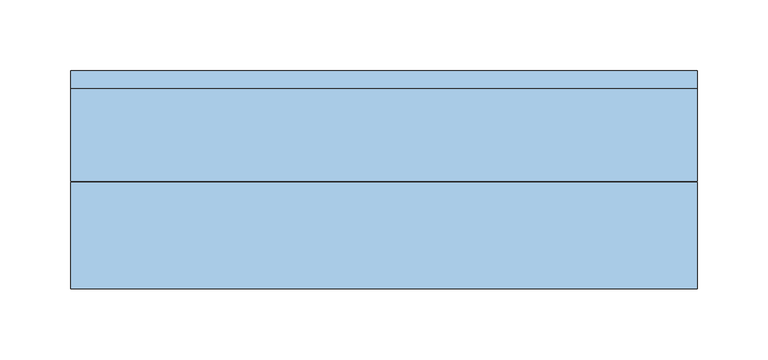
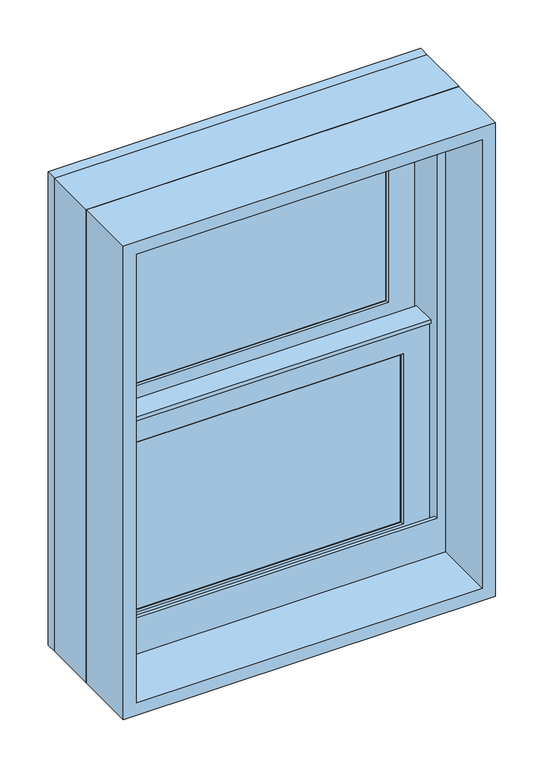
"""IFC4 building model written with IfcOpenShell, lengths in millimetres: window geometry, Window-Double_Hung-Marvin-Essential : ESDH1620."""

from ifc_helpers import new_model, si_unit, frame, origin, place, context, project, spatial, polyline, outline, extrude, faceted_brep, source, transform, mapped, element, save


def window_cd0364a2(model_context):
    return source(origin(), model_context, "Body", "SolidModel", [
        extrude(outline(polyline([(64.5583333, 20.6375), (64.5583333, 15.875), (45.5083333, 15.875), (45.5083333, 20.6375), (64.5583333, 20.6375)])), frame((0.0, 0.0, 1898.65), z_axis=(0.0, 0.0, 1.0), x_axis=(1.0, 0.0, 0.0)), (0.0, 0.0, 1.0), 222.25),
        extrude(outline(polyline([(-45.5083333, 20.6375), (-45.5083333, 15.875), (-64.5583333, 15.875), (-64.5583333, 20.6375), (-45.5083333, 20.6375)])), frame((0.0, 0.0, 1898.65), z_axis=(0.0, 0.0, 1.0), x_axis=(1.0, 0.0, 0.0)), (0.0, 0.0, 1.0), 222.25),
        extrude(outline(polyline([(165.1, 20.6375), (165.1, 15.875), (-165.1, 15.875), (-165.1, 20.6375), (165.1, 20.6375)])), frame((0.0, 0.0, 2000.25), z_axis=(0.0, 0.0, 1.0), x_axis=(1.0, 0.0, 0.0)), (0.0, 0.0, 1.0), 19.05),
        extrude(outline(polyline([(-64.5583333, 46.83125), (-64.5583333, 51.59375), (-45.5083333, 51.59375), (-45.5083333, 46.83125), (-64.5583333, 46.83125)])), frame((0.0, 0.0, 2159.0), z_axis=(0.0, 0.0, 1.0), x_axis=(1.0, 0.0, 0.0)), (0.0, 0.0, 1.0), 222.25),
        extrude(outline(polyline([(45.5083333, 46.83125), (45.5083333, 51.59375), (64.5583333, 51.59375), (64.5583333, 46.83125), (45.5083333, 46.83125)])), frame((0.0, 0.0, 2159.0), z_axis=(0.0, 0.0, 1.0), x_axis=(1.0, 0.0, 0.0)), (0.0, 0.0, 1.0), 222.25),
        extrude(outline(polyline([(-165.1, 46.83125), (-165.1, 51.59375), (165.1, 51.59375), (165.1, 46.83125), (-165.1, 46.83125)])), frame((0.0, 0.0, 2260.6), z_axis=(0.0, 0.0, 1.0), x_axis=(1.0, 0.0, 0.0)), (0.0, 0.0, 1.0), 19.05),
        extrude(outline(polyline([(64.5583333, 20.6375), (45.5083333, 20.6375), (45.5083333, 25.4), (64.5583333, 25.4), (64.5583333, 20.6375)])), frame((0.0, 0.0, 1898.65), z_axis=(0.0, 0.0, 1.0), x_axis=(1.0, 0.0, 0.0)), (0.0, 0.0, 1.0), 222.25),
        extrude(outline(polyline([(-45.5083333, 20.6375), (-64.5583333, 20.6375), (-64.5583333, 25.4), (-45.5083333, 25.4), (-45.5083333, 20.6375)])), frame((0.0, 0.0, 1898.65), z_axis=(0.0, 0.0, 1.0), x_axis=(1.0, 0.0, 0.0)), (0.0, 0.0, 1.0), 222.25),
        extrude(outline(polyline([(165.1, 20.6375), (-165.1, 20.6375), (-165.1, 25.4), (165.1, 25.4), (165.1, 20.6375)])), frame((0.0, 0.0, 2000.25), z_axis=(0.0, 0.0, 1.0), x_axis=(1.0, 0.0, 0.0)), (0.0, 0.0, 1.0), 19.05),
        extrude(outline(polyline([(-64.5583333, 56.35625), (-45.5083333, 56.35625), (-45.5083333, 51.59375), (-64.5583333, 51.59375), (-64.5583333, 56.35625)])), frame((0.0, 0.0, 2159.0), z_axis=(0.0, 0.0, 1.0), x_axis=(1.0, 0.0, 0.0)), (0.0, 0.0, 1.0), 222.25),
        extrude(outline(polyline([(45.5083333, 56.35625), (64.5583333, 56.35625), (64.5583333, 51.59375), (45.5083333, 51.59375), (45.5083333, 56.35625)])), frame((0.0, 0.0, 2159.0), z_axis=(0.0, 0.0, 1.0), x_axis=(1.0, 0.0, 0.0)), (0.0, 0.0, 1.0), 222.25),
        extrude(outline(polyline([(-165.1, 56.35625), (165.1, 56.35625), (165.1, 51.59375), (-165.1, 51.59375), (-165.1, 56.35625)])), frame((0.0, 0.0, 2260.6), z_axis=(0.0, 0.0, 1.0), x_axis=(1.0, 0.0, 0.0)), (0.0, 0.0, 1.0), 19.05),
        faceted_brep([(-192.0875, 5.6780605, 2150.9351748), (-192.0875, 5.6780605, 2146.3), (192.0875, 5.6780605, 2146.3), (192.0875, 5.6780605, 2150.9351748), (-192.0875, 34.8118605, 2150.9351748), (192.0875, 34.8118605, 2150.9351748), (192.0875, 34.8118605, 2146.3), (-192.0875, 34.8118605, 2146.3), (-192.0875, 30.1625, 2146.3), (-192.0875, 30.1625, 1871.6625), (-192.0875, 8.9241104, 1871.6625), (-192.0875, 8.9241104, 2146.3), (192.0875, 8.9241104, 2146.3), (192.0875, 30.1625, 2146.3), (192.0875, 8.9241104, 1871.6625), (192.0875, 30.1625, 1871.6625), (-176.2034752, 11.90625, 2132.0034752), (-176.2034752, 30.1625, 2132.0034752), (176.2034752, 30.1625, 2132.0034752), (176.2034752, 11.90625, 2132.0034752), (-159.54375, 10.4662439, 2115.34375), (-159.54375, 11.90625, 2115.34375), (159.54375, 11.90625, 2115.34375), (159.54375, 10.4662439, 2115.34375), (161.0858834, 8.9241104, 2116.8858834), (-161.0858834, 8.9241104, 2116.8858834), (176.2034752, 30.1625, 1887.5465248), (176.2034752, 11.90625, 1887.5465248), (159.54375, 11.90625, 1904.20625), (159.54375, 10.4662439, 1904.20625), (161.0858834, 8.9241104, 1902.6641166), (-176.2034752, 30.1625, 1887.5465248), (-176.2034752, 11.90625, 1887.5465248), (-159.54375, 11.90625, 1904.20625), (-159.54375, 10.4662439, 1904.20625), (-161.0858834, 8.9241104, 1902.6641166)], [[[0, 1, 2, 3]], [[4, 5, 6, 7]], [[1, 0, 4, 7, 8, 9, 10, 11]], [[2, 1, 11, 12]], [[7, 6, 13, 8]], [[3, 2, 12, 14, 15, 13, 6, 5]], [[0, 3, 5, 4]], [[16, 17, 18, 19]], [[20, 21, 22, 23]], [[20, 23, 24, 25]], [[19, 18, 26, 27]], [[23, 22, 28, 29]], [[24, 23, 29, 30]], [[27, 26, 31, 32]], [[29, 28, 33, 34]], [[30, 29, 34, 35]], [[15, 14, 10, 9]], [[15, 9, 8, 13], [18, 17, 31, 26]], [[17, 16, 32, 31]], [[16, 19, 27, 32], [22, 21, 33, 28]], [[21, 20, 34, 33]], [[20, 25, 35, 34]], [[10, 14, 12, 11], [25, 24, 30, 35]]]),
        extrude(outline(polyline([(38.5955581, 2132.0125), (33.5778968, 2132.0125), (33.5778968, 2133.6), (39.9405976, 2133.6), (39.9405976, 2132.0125), (61.515625, 2132.0125), (47.6307501, 2128.6975159), (38.5955581, 2128.6975159), (38.5955581, 2132.0125)])), frame((-192.0875, 0.0, 0.0), z_axis=(1.0, 0.0, 0.0), x_axis=(0.0, 1.0, 0.0)), (0.0, 0.0, 1.0), 384.175),
        faceted_brep([(222.25, 0.0, 1841.5), (222.25, 0.0, 2438.4), (-222.25, 0.0, 2438.4), (-222.25, 0.0, 1841.5), (196.05625, 0.0, 1902.61875), (-196.05625, 0.0, 1902.61875), (-196.05625, 0.0, 2412.20625), (196.05625, 0.0, 2412.20625), (196.05625, 3.96875, 1841.5), (-196.05625, 3.96875, 1841.5), (-196.05625, 3.96875, 1902.61875), (196.05625, 3.96875, 1902.61875), (-222.25, 65.6828125, 1841.5), (-196.05625, 65.6828125, 1841.5), (196.05625, 65.6828125, 1841.5), (222.25, 65.6828125, 1841.5), (-222.25, 65.6828125, 2438.4), (222.25, 65.6828125, 2438.4), (196.05625, 65.6828125, 2412.20625), (-196.05625, 65.6828125, 2412.20625)], [[[0, 1, 2, 3], [4, 5, 6, 7]], [[8, 9, 10, 11]], [[5, 4, 11, 10]], [[0, 3, 12, 13, 9, 8, 14, 15]], [[13, 12, 16, 17, 15, 14, 18, 19]], [[13, 19, 6, 5, 10, 9]], [[7, 6, 19, 18]], [[18, 14, 8, 11, 4, 7]], [[1, 0, 15, 17]], [[2, 1, 17, 16]], [[3, 2, 16, 12]]]),
        faceted_brep([(196.05625, 30.1625, 2139.95), (194.46875, 30.1625, 2139.95), (194.46875, 30.1625, 1865.8544613), (196.05625, 30.1625, 1865.8544613), (-194.46875, 30.1625, 2139.95), (-196.05625, 30.1625, 2139.95), (-196.05625, 30.1625, 1865.8544613), (-194.46875, 30.1625, 1865.8544613), (194.46875, 63.5, 2139.95), (196.05625, 63.5, 2139.95), (196.05625, 63.5, 1859.3743077), (194.46875, 63.5, 1859.3743077), (-196.05625, 63.5, 2139.95), (-194.46875, 63.5, 2139.95), (-194.46875, 63.5, 1859.3743077), (-196.05625, 63.5, 1859.3743077), (207.3108932, 3.96875, 1870.9460105), (207.3108932, 3.96875, 1841.5), (207.3108932, 65.6828125, 1841.5), (207.3108932, 65.6828125, 1858.950012), (-207.3108932, 3.96875, 1841.5), (-207.3108932, 3.96875, 1870.9460105), (-207.3108932, 65.6828125, 1858.950012), (-207.3108932, 65.6828125, 1841.5), (207.3108932, 78.58125, 1856.4428097), (-207.3108932, 78.58125, 1856.4428097), (-205.2971252, 68.2348864, 1858.4539391), (-187.33135, 68.2348864, 1858.4539391), (-187.33135, 65.6828125, 1858.950012), (187.33135, 65.6828125, 1858.950012), (187.33135, 68.2348864, 1858.4539391), (205.2971252, 68.2348864, 1858.4539391), (-222.25, 65.6828125, 1841.5), (-222.25, 78.5948249, 1841.5), (222.25, 78.5948249, 1841.5), (222.25, 65.6828125, 1841.5), (-222.25, 78.58125, 2438.4), (222.25, 78.58125, 2438.4), (207.3108932, 78.58125, 2423.4608932), (-207.3108932, 78.58125, 2423.4608932), (-222.25, 65.6828125, 2438.4), (-205.2971252, 68.2348864, 2421.4471252), (205.2971252, 68.2348864, 2421.4471252), (187.33135, 68.2348864, 2403.48135), (-187.33135, 68.2348864, 2403.48135), (-187.33135, 65.6828125, 2403.48135), (187.33135, 65.6828125, 2403.48135), (222.25, 65.6828125, 2438.4)], [[[0, 1, 2, 3]], [[4, 5, 6, 7]], [[8, 9, 10, 11]], [[12, 13, 14, 15]], [[1, 8, 11, 2]], [[9, 0, 3, 10]], [[1, 0, 9, 8]], [[5, 4, 13, 12]], [[5, 12, 15, 6]], [[13, 4, 7, 14]], [[16, 17, 18, 19]], [[20, 21, 22, 23]], [[24, 25, 26, 27, 28, 22, 21, 16, 19, 29, 30, 31], [3, 2, 11, 10], [7, 6, 15, 14]], [[17, 16, 21, 20]], [[17, 20, 23, 32, 33, 34, 35, 18]], [[34, 33, 36, 37], [25, 24, 38, 39]], [[33, 32, 40, 36]], [[39, 41, 26, 25]], [[41, 42, 31, 30, 43, 44, 27, 26]], [[44, 45, 28, 27]], [[40, 32, 23, 22, 28, 45, 46, 29, 19, 18, 35, 47]], [[36, 40, 47, 37]], [[39, 38, 42, 41]], [[44, 43, 46, 45]], [[34, 37, 47, 35]], [[42, 38, 24, 31]], [[46, 43, 30, 29]]]),
        extrude(outline(polyline([(172.24375, 11.90625), (-172.24375, 11.90625), (-172.24375, 15.08125), (172.24375, 15.08125), (172.24375, 11.90625)])), frame((0.0, 0.0, 1891.50625), z_axis=(0.0, 0.0, 1.0), x_axis=(1.0, 0.0, 0.0)), (0.0, 0.0, 1.0), 236.5375),
        extrude(outline(polyline([(172.24375, 42.8625), (-172.24375, 42.8625), (-172.24375, 46.0375), (172.24375, 46.0375), (172.24375, 42.8625)])), frame((0.0, 0.0, 2151.85625), z_axis=(0.0, 0.0, 1.0), x_axis=(1.0, 0.0, 0.0)), (0.0, 0.0, 1.0), 236.5375),
        faceted_brep([(-159.54375, 31.194477, 2115.34375), (-161.0858834, 32.7366104, 2116.8858834), (161.0858834, 32.7366104, 2116.8858834), (159.54375, 31.194477, 2115.34375), (-159.54375, 30.1625, 2115.34375), (159.54375, 30.1625, 2115.34375), (-192.0875, 32.7366104, 2147.8875), (-192.0875, 30.1625, 2147.8875), (192.0875, 30.1625, 2147.8875), (192.0875, 32.7366104, 2147.8875), (161.0858834, 32.7366104, 1902.6641166), (159.54375, 31.194477, 1904.20625), (159.54375, 30.1625, 1904.20625), (192.0875, 30.1625, 1871.6625), (192.0875, 32.7366104, 1871.6625), (-161.0858834, 32.7366104, 1902.6641166), (-159.54375, 31.194477, 1904.20625), (-159.54375, 30.1625, 1904.20625), (-192.0875, 30.1625, 1871.6625), (-192.0875, 32.7366104, 1871.6625)], [[[0, 1, 2, 3]], [[4, 0, 3, 5]], [[6, 7, 8, 9]], [[3, 2, 10, 11]], [[5, 3, 11, 12]], [[9, 8, 13, 14]], [[11, 10, 15, 16]], [[12, 11, 16, 17]], [[14, 13, 18, 19]], [[9, 14, 19, 6], [1, 15, 10, 2]], [[16, 15, 1, 0]], [[17, 16, 0, 4]], [[7, 18, 13, 8], [5, 12, 17, 4]], [[19, 18, 7, 6]]]),
        faceted_brep([(-176.2034752, 42.8625, 2392.3534752), (-176.2034752, 61.11875, 2392.3534752), (176.2034752, 61.11875, 2392.3534752), (176.2034752, 42.8625, 2392.3534752), (-159.54375, 41.4224939, 2375.69375), (-159.54375, 42.8625, 2375.69375), (159.54375, 42.8625, 2375.69375), (159.54375, 41.4224939, 2375.69375), (-161.0858834, 39.8803604, 2377.2358834), (161.0858834, 39.8803604, 2377.2358834), (-192.0875, 61.11875, 2408.2375), (-192.0875, 39.8803604, 2408.2375), (192.0875, 39.8803604, 2408.2375), (192.0875, 61.11875, 2408.2375), (176.2034752, 61.11875, 2147.8965248), (176.2034752, 42.8625, 2147.8965248), (159.54375, 42.8625, 2164.55625), (159.54375, 41.4224939, 2164.55625), (161.0858834, 39.8803604, 2163.0141166), (192.0875, 39.8803604, 2132.0125), (192.0875, 61.11875, 2132.0125), (-176.2034752, 61.11875, 2147.8965248), (-176.2034752, 42.8625, 2147.8965248), (-159.54375, 42.8625, 2164.55625), (-159.54375, 41.4224939, 2164.55625), (-161.0858834, 39.8803604, 2163.0141166), (-192.0875, 39.8803604, 2132.0125), (-192.0875, 61.11875, 2132.0125)], [[[0, 1, 2, 3]], [[4, 5, 6, 7]], [[8, 4, 7, 9]], [[10, 11, 12, 13]], [[3, 2, 14, 15]], [[7, 6, 16, 17]], [[9, 7, 17, 18]], [[13, 12, 19, 20]], [[15, 14, 21, 22]], [[17, 16, 23, 24]], [[18, 17, 24, 25]], [[20, 19, 26, 27]], [[13, 20, 27, 10], [1, 21, 14, 2]], [[22, 21, 1, 0]], [[3, 15, 22, 0], [5, 23, 16, 6]], [[24, 23, 5, 4]], [[25, 24, 4, 8]], [[11, 26, 19, 12], [9, 18, 25, 8]], [[27, 26, 11, 10]]]),
        faceted_brep([(-192.0875, 61.11875, 2132.0125), (-192.0875, 63.6928604, 2132.0125), (192.0875, 63.6928604, 2132.0125), (192.0875, 61.11875, 2132.0125), (-159.54375, 62.150727, 2164.55625), (-159.54375, 61.11875, 2164.55625), (159.54375, 61.11875, 2164.55625), (159.54375, 62.150727, 2164.55625), (-161.0858834, 63.6928604, 2163.0141166), (161.0858834, 63.6928604, 2163.0141166), (192.0875, 63.6928604, 2408.2375), (192.0875, 61.11875, 2408.2375), (159.54375, 61.11875, 2375.69375), (159.54375, 62.150727, 2375.69375), (161.0858834, 63.6928604, 2377.2358834), (-192.0875, 63.6928604, 2408.2375), (-192.0875, 61.11875, 2408.2375), (-159.54375, 61.11875, 2375.69375), (-159.54375, 62.150727, 2375.69375), (-161.0858834, 63.6928604, 2377.2358834)], [[[0, 1, 2, 3]], [[4, 5, 6, 7]], [[8, 4, 7, 9]], [[3, 2, 10, 11]], [[7, 6, 12, 13]], [[9, 7, 13, 14]], [[11, 10, 15, 16]], [[13, 12, 17, 18]], [[14, 13, 18, 19]], [[16, 15, 1, 0]], [[3, 11, 16, 0], [5, 17, 12, 6]], [[18, 17, 5, 4]], [[19, 18, 4, 8]], [[1, 15, 10, 2], [9, 14, 19, 8]]]),
        extrude(outline(polyline([(172.24375, 26.19375), (-172.24375, 26.19375), (-172.24375, 30.1625), (172.24375, 30.1625), (172.24375, 26.19375)])), frame((0.0, 0.0, 1891.50625), z_axis=(0.0, 0.0, 1.0), x_axis=(1.0, 0.0, 0.0)), (0.0, 0.0, 1.0), 236.5375),
        extrude(outline(polyline([(172.24375, 57.15), (-172.24375, 57.15), (-172.24375, 61.11875), (172.24375, 61.11875), (172.24375, 57.15)])), frame((0.0, 0.0, 2151.85625), z_axis=(0.0, 0.0, 1.0), x_axis=(1.0, 0.0, 0.0)), (0.0, 0.0, 1.0), 236.5375),
        extrude(outline(polyline([(2438.4, 222.25), (2438.4, -222.25), (1841.5, -222.25), (1841.5, 222.25), (2438.4, 222.25)]), holes=[polyline([(2422.525, 206.375), (1857.375, 206.375), (1857.375, -206.375), (2422.525, -206.375), (2422.525, 206.375)])]), frame((0.0, -76.2, 0.0), z_axis=(0.0, 1.0, 0.0), x_axis=(0.0, 0.0, 1.0)), (0.0, 0.0, 1.0), 75.40625),
    ])


if __name__ == "__main__":
    model = new_model("IFC4")
    model_context = context("Model", 3, world=origin())
    ifc_project = project(units=[si_unit("LENGTHUNIT", "METRE", prefix="MILLI")], contexts=[model_context])
    site = spatial("IfcSite", under=ifc_project)
    building = spatial("IfcBuilding", under=site)
    placement = place(None, origin())
    window_shape = window_cd0364a2(model_context)
    element("IfcWindow", 1, ObjectType="Window-Double_Hung-Marvin-Essential : ESDH1620", at=placement, inside=building, context=model_context, shape_type="MappedRepresentation", body=[
        mapped(window_shape, transform((0.0, 0.0, 0.0), x_axis=(1.0, 0.0, 0.0), y_axis=(0.0, 1.0, 0.0), z_axis=(0.0, 0.0, 1.0))),
    ])
    save(model, "model.ifc")

# Revit data of these elements
# Type "Window-Double_Hung-Marvin-Essential : ESDH1620"
#   Type Mark = "19"
#   Window Type = "Essential Double Hung"
#   Product data url = "https://bimobject.com/marvin-windows-and-doors/product/marvin-dhwau"
#   Product Guid = "c4a96547-874c-4385-91dc-a058adc19d98"
#   Frame = "All Ultrex"
#   Egress Window = "No"
#   URL = "www.marvin.com"
#   Model = "ESDH1620"
#   Manufacturer = "Marvin Windows and Doors"
#   Label Egress = ""
#   Glass Type = "IG Low E II with Argon"
#   Design Pressure = "DP50"
#   Description = "1824 DBHG"
#   Analytic Construction = "<None>"
#   Prairie Corner Width = 0' - 4"
#   Prairie Corner Height = 0' - 4"
#   Egress Width = 1' - 2 9/16"
#   Egress Height = 0' - 7 27/128"
#   Rough Width = 1' - 6"
#   Rough Height = 2' - 0"
#   Nominal Width = 1' - 6"
#   Nominal Height = 2' - 0"
#   Inset to Installation Flange [instance default] = 0' - 1"
#   Height = 1' - 11 1/2"
#   Egress Area = 0.729231 SF
#   Default Head Height = 8' - 0"
#   Width = 1' - 5 1/2"
#   Daylight Area = 1.45036 SF
#   DLO Width = 1' - 0 9/16"
#   DLO Height = 0' - 8 5/16"
#   Muntins Top Sash = yes
#   Lites Wide Top Sash = 3
#   Lites Wide Bottom Sash = 3
#   Lites High Top Sash = 2
#   Lites High Bottom Sash = 2
#   Lite Cut Prairie 9 = no
#   Lite Cut HV Grid = yes
#   Muntins Bottom Sash = yes
#   Label Visibility = no
#   Jamb Extension Visibility = yes
#   Edition number = 1
#   Interior Material = Ultrex-Marvin-Stonewhite
#   Glazing Material = Glass-Marvin-IG Low E II with Argon
#   Cladding Material = Ultrex-Marvin-Pebblegray
#   Wall Closure = (empty or 0)
#   Assembly Code = ""
# Element 1 (IfcWindow, "Window-Double_Hung-Marvin-Essential : ESDH1620")
#   Materials on its faces: "Ultrex-Marvin-Pebblegray", "Ultrex-Marvin-Stonewhite", "Glass-Marvin-IG Low E II with Argon"
# Materials
#   "Ultrex-Marvin-Stonewhite": class "Paint", colour RGB 250 251 245, transparency 0
#   "Glass-Marvin-IG Low E II with Argon": class "Glass", colour RGB 0 128 192, transparency 0.85
#   "Ultrex-Marvin-Pebblegray": class "Paint", colour RGB 189 185 173, transparency 0
